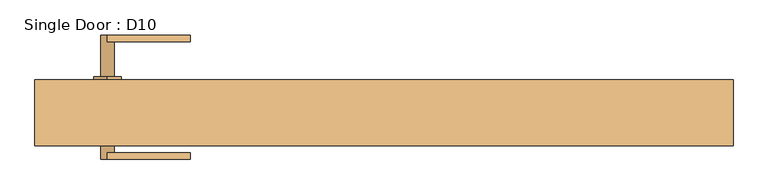
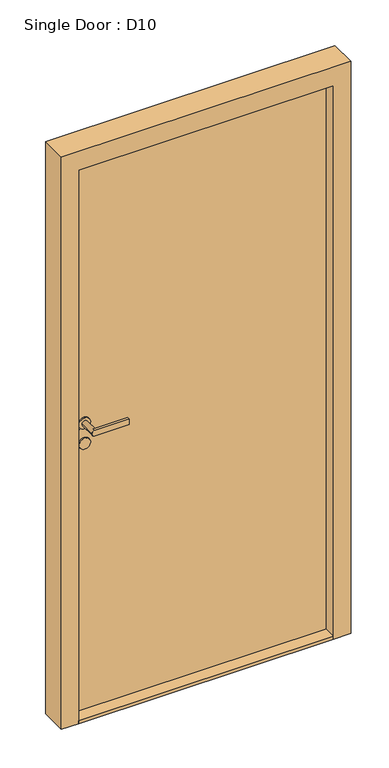
"""IFC4 building model written with IfcOpenShell, lengths in millimetres: door geometry, Single Door : D10."""

from ifc_helpers import new_model, si_unit, point, frame, frame_2d, origin, origin_with_axes, place, context, project, spatial, polyline, circle_curve, trimmed, segment, composite_curve, outline, extrude, source, transform, mapped, element, save
from ifc_brep_helpers import plane_surface, cylinder_surface, advanced_brep


def single_door_d10_bed63a48(model_context):
    return source(origin(), model_context, "Body", "SolidModel", [
        advanced_brep(
        [(-400.0, -5.0, 1057.5), (-390.0, -5.0, 1067.5), (-400.0, -5.0, 1077.5), (-280.0, -5.0, 1077.5), (-280.0, -5.0, 1057.5), (-400.0, -15.0, 1077.5), (-410.0, -15.0, 1067.5), (-400.0, -15.0, 1057.5), (-280.0, -15.0, 1057.5), (-280.0, -15.0, 1077.5), (-390.0, 45.0, 1067.5), (-410.0, 45.0, 1067.5)],
        [
            (0, 1, circle_curve(frame((-400.0, -5.0, 1067.5), z_axis=(0.0, -1.0, 0.0), x_axis=(0.0, 0.0, 1.0)), 10.0)),
            (1, 2, circle_curve(frame((-400.0, -5.0, 1067.5), z_axis=(0.0, -1.0, 0.0), x_axis=(0.0, 0.0, 1.0)), 10.0)),
            (2, 3),
            (3, 4),
            (4, 0),
            (5, 6, circle_curve(frame((-400.0, -15.0, 1067.5), z_axis=(0.0, -1.0, 0.0), x_axis=(0.0, 0.0, 1.0)), 10.0)),
            (6, 7, circle_curve(frame((-400.0, -15.0, 1067.5), z_axis=(0.0, -1.0, 0.0), x_axis=(0.0, 0.0, 1.0)), 10.0)),
            (7, 8),
            (8, 9),
            (9, 5),
            (4, 8),
            (7, 0),
            (3, 9),
            (2, 5),
            (10, 11, circle_curve(frame((-400.0, 45.0, 1067.5), z_axis=(0.0, 1.0, 0.0), x_axis=(0.0, 0.0, 1.0)), 10.0)),
            (11, 10, circle_curve(frame((-400.0, 45.0, 1067.5), z_axis=(0.0, 1.0, 0.0), x_axis=(0.0, 0.0, 1.0)), 10.0)),
            (11, 6),
            (1, 10),
        ],
        [
            plane_surface(frame((-400.0, -5.0, 1057.5), z_axis=(0.0, 1.0, 0.0), x_axis=(1.0, 0.0, 0.0))),
            plane_surface(frame((-400.0, -15.0, 1057.5), z_axis=(0.0, -1.0, 0.0), x_axis=(-1.0, 0.0, 0.0))),
            plane_surface(frame((-400.0, -5.0, 1057.5), z_axis=(0.0, 0.0, -1.0), x_axis=(0.0, -1.0, 0.0))),
            plane_surface(frame((-280.0, -5.0, 1057.5), z_axis=(1.0, 0.0, 0.0), x_axis=(0.0, -1.0, 0.0))),
            plane_surface(frame((-280.0, -5.0, 1077.5), z_axis=(0.0, 0.0, 1.0), x_axis=(0.0, -1.0, 0.0))),
            plane_surface(frame((-400.0, 45.0, 1077.5), z_axis=(0.0, 1.0, 0.0), x_axis=(-1.0, 0.0, 0.0))),
            cylinder_surface(frame((-400.0, -15.0, 1067.5), z_axis=(0.0, 1.0, 0.0), x_axis=(0.0, 0.0, 1.0)), 10.0),
        ],
        [
            (0, [[1, 2, 3, 4, 5]]),
            (1, [[6, 7, 8, 9, 10]]),
            (2, [[11, -8, 12, -5]]),
            (3, [[13, -9, -11, -4]]),
            (4, [[14, -10, -13, -3]]),
            (5, [[15, 16]]),
            (6, [[17, -6, -14, -2, 18, -16]]),
            (6, [[-18, -1, -12, -7, -17, -15]]),
        ],
    ),
        advanced_brep(
        [(-400.0, 165.0, 1057.5), (-410.0, 165.0, 1067.5), (-400.0, 165.0, 1077.5), (-280.0, 165.0, 1077.5), (-280.0, 165.0, 1057.5), (-400.0, 155.0, 1077.5), (-390.0, 155.0, 1067.5), (-400.0, 155.0, 1057.5), (-280.0, 155.0, 1057.5), (-280.0, 155.0, 1077.5), (-410.0, 105.0, 1067.5), (-390.0, 105.0, 1067.5)],
        [
            (0, 1, circle_curve(frame((-400.0, 165.0, 1067.5), z_axis=(0.0, 1.0, 0.0), x_axis=(1.0, 0.0, 0.0)), 10.0)),
            (1, 2, circle_curve(frame((-400.0, 165.0, 1067.5), z_axis=(0.0, 1.0, 0.0), x_axis=(1.0, 0.0, 0.0)), 10.0)),
            (2, 3),
            (3, 4),
            (4, 0),
            (5, 6, circle_curve(frame((-400.0, 155.0, 1067.5), z_axis=(0.0, 1.0, 0.0), x_axis=(1.0, 0.0, 0.0)), 10.0)),
            (6, 7, circle_curve(frame((-400.0, 155.0, 1067.5), z_axis=(0.0, 1.0, 0.0), x_axis=(1.0, 0.0, 0.0)), 10.0)),
            (7, 8),
            (8, 9),
            (9, 5),
            (4, 8),
            (7, 0),
            (3, 9),
            (2, 5),
            (10, 11, circle_curve(frame((-400.0, 105.0, 1067.5), z_axis=(0.0, -1.0, 0.0), x_axis=(1.0, 0.0, 0.0)), 10.0)),
            (11, 10, circle_curve(frame((-400.0, 105.0, 1067.5), z_axis=(0.0, -1.0, 0.0), x_axis=(1.0, 0.0, 0.0)), 10.0)),
            (10, 1),
            (6, 11),
        ],
        [
            plane_surface(frame((-400.0, 165.0, 1057.5), z_axis=(0.0, 1.0, 0.0), x_axis=(1.0, 0.0, 0.0))),
            plane_surface(frame((-400.0, 155.0, 1057.5), z_axis=(0.0, -1.0, 0.0), x_axis=(-1.0, 0.0, 0.0))),
            plane_surface(frame((-400.0, 165.0, 1057.5), z_axis=(0.0, 0.0, -1.0), x_axis=(0.0, -1.0, 0.0))),
            plane_surface(frame((-280.0, 165.0, 1057.5), z_axis=(1.0, 0.0, 0.0), x_axis=(0.0, -1.0, 0.0))),
            plane_surface(frame((-280.0, 165.0, 1077.5), z_axis=(0.0, 0.0, 1.0), x_axis=(0.0, -1.0, 0.0))),
            plane_surface(frame((-390.0, 105.0, 1067.5), z_axis=(0.0, -1.0, 0.0), x_axis=(0.0, 0.0, -1.0))),
            cylinder_surface(frame((-400.0, 105.0, 1067.5), z_axis=(0.0, 1.0, 0.0), x_axis=(1.0, 0.0, 0.0)), 10.0),
        ],
        [
            (0, [[1, 2, 3, 4, 5]]),
            (1, [[6, 7, 8, 9, 10]]),
            (2, [[11, -8, 12, -5]]),
            (3, [[13, -9, -11, -4]]),
            (4, [[14, -10, -13, -3]]),
            (5, [[15, 16]]),
            (6, [[17, -1, -12, -7, 18, -15]]),
            (6, [[-18, -6, -14, -2, -17, -16]]),
        ],
    ),
        extrude(outline(composite_curve([segment(trimmed(circle_curve(frame_2d((1067.5, -400.0)), 20.0), [point((1047.5, -400.0))], [point((1087.5, -400.0))], False, "CARTESIAN"), True, "CONTINUOUS"), segment(trimmed(circle_curve(frame_2d((1067.5, -400.0)), 20.0), [point((1087.5, -400.0))], [point((1047.5, -400.0))], False, "CARTESIAN"), True, "CONTINUOUS")], self_intersect=False)), frame((0.0, 45.0, 0.0), z_axis=(0.0, 1.0, 0.0), x_axis=(0.0, 0.0, 1.0)), (0.0, 0.0, 1.0), 5.0),
        extrude(outline(composite_curve([segment(trimmed(circle_curve(frame_2d((992.5, -400.0)), 20.0), [point((972.5, -400.0))], [point((1012.5, -400.0))], False, "CARTESIAN"), True, "CONTINUOUS"), segment(trimmed(circle_curve(frame_2d((992.5, -400.0)), 20.0), [point((1012.5, -400.0))], [point((972.5, -400.0))], False, "CARTESIAN"), True, "CONTINUOUS")], self_intersect=False)), frame((0.0, 45.0, 0.0), z_axis=(0.0, 1.0, 0.0), x_axis=(0.0, 0.0, 1.0)), (0.0, 0.0, 1.0), 5.0),
        extrude(outline(composite_curve([segment(trimmed(circle_curve(frame_2d((1067.5, -400.0)), 20.0), [point((1047.5, -400.0))], [point((1087.5, -400.0))], False, "CARTESIAN"), True, "CONTINUOUS"), segment(trimmed(circle_curve(frame_2d((1067.5, -400.0)), 20.0), [point((1087.5, -400.0))], [point((1047.5, -400.0))], False, "CARTESIAN"), True, "CONTINUOUS")], self_intersect=False)), frame((0.0, 100.0, 0.0), z_axis=(0.0, 1.0, 0.0), x_axis=(0.0, 0.0, 1.0)), (0.0, 0.0, 1.0), 5.0),
        extrude(outline(composite_curve([segment(trimmed(circle_curve(frame_2d((992.5, -400.0)), 20.0), [point((972.5, -400.0))], [point((1012.5, -400.0))], False, "CARTESIAN"), True, "CONTINUOUS"), segment(trimmed(circle_curve(frame_2d((992.5, -400.0)), 20.0), [point((1012.5, -400.0))], [point((972.5, -400.0))], False, "CARTESIAN"), True, "CONTINUOUS")], self_intersect=False)), frame((0.0, 100.0, 0.0), z_axis=(0.0, 1.0, 0.0), x_axis=(0.0, 0.0, 1.0)), (0.0, 0.0, 1.0), 5.0),
        extrude(outline(polyline([(445.0, 50.0), (-445.0, 50.0), (-445.0, 100.0), (445.0, 100.0), (445.0, 50.0)])), frame((0.0, 0.0, 10.0), z_axis=(0.0, 0.0, 1.0), x_axis=(1.0, 0.0, 0.0)), (0.0, 0.0, 1.0), 2030.0),
        extrude(outline(polyline([(2110.0, 505.0), (2110.0, -505.0), (0.0, -505.0), (0.0, -445.0), (2040.0, -445.0), (2040.0, 445.0), (0.0, 445.0), (0.0, 505.0), (2110.0, 505.0)])), frame((0.0, 5.0, 0.0), z_axis=(0.0, 1.0, 0.0), x_axis=(0.0, 0.0, 1.0)), (0.0, 0.0, 1.0), 95.0),
        extrude(outline(polyline([(-445.0, 5.0), (-445.0, 100.0), (445.0, 100.0), (445.0, 5.0), (-445.0, 5.0)])), origin_with_axes(), (0.0, 0.0, 1.0), 10.0),
    ])


if __name__ == "__main__":
    model = new_model("IFC4")
    model_context = context("Model", 3, world=origin())
    ifc_project = project(units=[si_unit("LENGTHUNIT", "METRE", prefix="MILLI")], contexts=[model_context])
    site = spatial("IfcSite", under=ifc_project)
    building = spatial("IfcBuilding", under=site)
    placement = place(None, origin())
    single_door_d10_shape = single_door_d10_bed63a48(model_context)
    element("IfcDoor", 1, ObjectType="Single Door : D10", at=placement, inside=building, context=model_context, shape_type="MappedRepresentation", body=[
        mapped(single_door_d10_shape, transform((0.0, 0.0, 0.0), x_axis=(1.0, 0.0, 0.0), y_axis=(0.0, 1.0, 0.0), z_axis=(0.0, 0.0, 1.0))),
    ])
    save(model, "model.ifc")

# Revit data of these elements
# Type "Single Door : D10"
#   Type Mark = "D10"
#   Fire Rating = "EI 120"
#   CQSwingCount = ""
#   CQTypeCount = ""
#   URL = "http://www.cad-q.com"
#   Keynote = "43.CC"
#   Construction Type = "Generell innerdörr"
#   CQOriginalSwingDirection = "Left"
#   Wall Width [instance default] = 200 mm
#   Thickness = 50 mm
#   Inset1000 [instance default] = 1000 mm
#   Inset [instance default] = 0 mm
#   GapTop [instance default] = 20 mm
#   GapLock [instance default] = 10 mm
#   GapHinge [instance default] = 10 mm
#   Gap = 10 mm
#   Frame Width = 990 mm
#   Frame Thickness = 50 mm
#   Frame Height = 2090 mm
#   Frame Depth [instance default] = 95 mm
#   Plan Swing Angle = 90.00°
#   Standard Frame Depth = 95 mm
#   Rough Width = 1010 mm
#   Rough Height = 2110 mm
#   Threshold Height = 10 mm
#   Height [instance default] = 2110 mm
#   Width [instance default] = 1010 mm
#   Panel Height = 2030 mm
#   Panel Width = 890 mm
#   Clear Opening Width [instance default] = 840 mm
#   Threshold = yes
#   MWidth [instance default] = 10
#   MHeight [instance default] = 21
#   Gap Top [instance default] = yes
#   Gap Lock Side [instance default] = yes
#   Gap Hinge Side [instance default] = yes
#   CQReversedRoomAssociation [instance default] = no
#   Material Threshold = none
#   Material Panel = none
#   Material Frame = none
#   Material Exterior = none
#   Handle = element 307872
#   Material Glass = none
#   Door Panel = element 307881
#   Material Hardware = none
#   Operation = ""
#   Wall Closure = (empty or 0)
#   Function = (empty or 0)
#   Assembly Code = ""
# Element 1 (IfcDoor, "Single Door : D10")
#   Wall Width = 300 mm
#   Inset1000 = 1050 mm
#   Inset = 50 mm
#   Materials on its faces: "Default Hardware", "Door - Frame/Mullion"
# Materials
#   "Default Hardware": class "Generic", colour RGB 127 127 127, transparency 0, Description = "Default Ironmomgery", Cost = 0
#   "Door - Frame/Mullion": class "Wood", colour RGB 212 179 113, transparency 0, Keynote = "L20", Cost = 0
